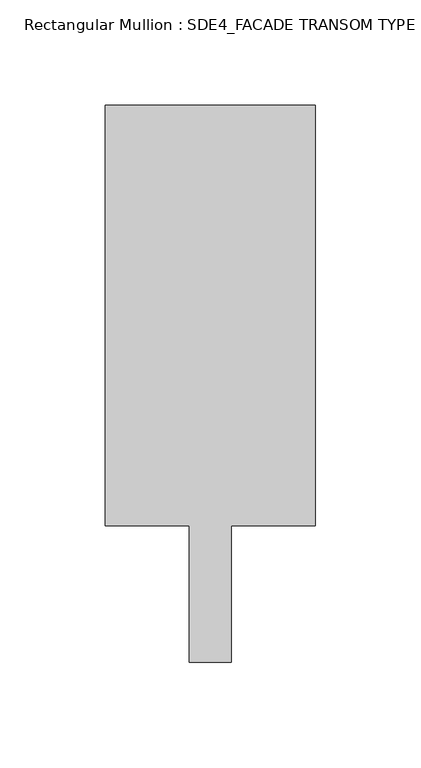
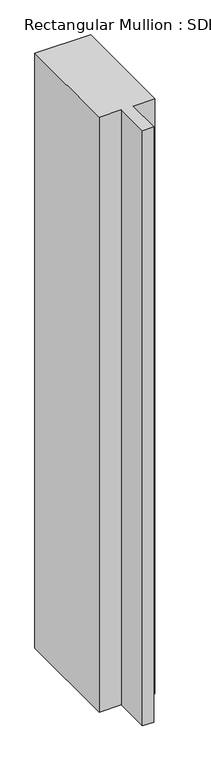
"""IFC4 building model written with IfcOpenShell, lengths in millimetres: member geometry, Rectangular Mullion : SDE4_FACADE TRANSOM TYPE 2."""

import ifcopenshell
import ifcopenshell.guid

model = None  # the IFC model being written
_history = None  # IfcOwnerHistory: only IFC2X3 demands one
_inside = {}  # id of a spatial element -> (the spatial element, [elements in it])
_under = {}  # id of a project, library or spatial element -> (it, [spatial elements below it])
_declared = {}  # id of a project -> (the project, [libraries it declares])
_typed = {}  # id of a type object -> (the type object, [elements of that type])
_made_of = {}  # id of a material, layer set ... -> (it, [elements and type objects made of it])


def new_model(schema):
    """Start an empty IFC model of exactly this schema.

    Asked for "IFC4X3", IfcOpenShell would pick the latest addendum, in which some entities
    have other attributes; the version numbers below select the first issue.
    IFC2X3 requires an IfcOwnerHistory on every rooted entity: one is made here for all.
    """
    global model, _history
    if schema == "IFC4X3":
        model = ifcopenshell.file(schema_version=(4, 3, 0, 0))
    else:
        model = ifcopenshell.file(schema=schema)
    _inside.clear()
    _under.clear()
    _declared.clear()
    _typed.clear()
    _made_of.clear()
    _history = None
    if model.schema == "IFC2X3":
        org = make("IfcOrganization", Name="unknown")
        user = make(
            "IfcPersonAndOrganization",
            ThePerson=make("IfcPerson", FamilyName="unknown"),
            TheOrganization=org,
        )
        app = make(
            "IfcApplication",
            ApplicationDeveloper=org,
            Version="unknown",
            ApplicationFullName="unknown",
            ApplicationIdentifier="unknown",
        )
        _history = make(
            "IfcOwnerHistory",
            OwningUser=user,
            OwningApplication=app,
            ChangeAction="ADDED",
            CreationDate=0,
        )
    return model


def make(cls, **values):
    """One entity of the class cls with the attributes given. An attribute that is None is left unset."""
    return model.create_entity(
        cls, **{name: value for name, value in values.items() if value is not None}
    )


def rooted(cls, **values):
    """An entity with a GlobalId (a new one), such as an element, a storey or a relation."""
    return make(cls, GlobalId=ifcopenshell.guid.new(), OwnerHistory=_history, **values)


def si_unit(unit_type, name, prefix=None):
    """IfcSIUnit, for example si_unit("LENGTHUNIT", "METRE", prefix="MILLI")."""
    return make("IfcSIUnit", UnitType=unit_type, Prefix=prefix, Name=name)


def assignment(units):
    """IfcUnitAssignment: the units of a project."""
    return None if units is None else make("IfcUnitAssignment", Units=units)


def point(xyz):
    """IfcCartesianPoint."""
    return None if xyz is None else make("IfcCartesianPoint", Coordinates=xyz)


def direction(xyz):
    """IfcDirection."""
    return None if xyz is None else make("IfcDirection", DirectionRatios=xyz)


def frame(location, z_axis=None, x_axis=None):
    """IfcAxis2Placement3D, a coordinate frame: its origin and axes. An axis left out is left unset."""
    return make(
        "IfcAxis2Placement3D",
        Location=point(location),
        Axis=direction(z_axis),
        RefDirection=direction(x_axis),
    )


def origin():
    """The frame at (0, 0, 0) with its axes left unset."""
    return frame((0.0, 0.0, 0.0))


def place(relative_to, where):
    """IfcLocalPlacement: puts the frame where relative to a parent placement (None: the world)."""
    return make(
        "IfcLocalPlacement", PlacementRelTo=relative_to, RelativePlacement=where
    )


def context(
    kind, dimensions, precision=None, world=None, true_north=None, identifier=None
):
    """IfcGeometricRepresentationContext, for example the 3D "Model" context."""
    return make(
        "IfcGeometricRepresentationContext",
        ContextIdentifier=identifier,
        ContextType=kind,
        CoordinateSpaceDimension=dimensions,
        Precision=precision,
        WorldCoordinateSystem=world,
        TrueNorth=true_north,
    )


def project(units=None, contexts=None):
    """IfcProject with its units and contexts."""
    return rooted(
        "IfcProject",
        Name="project",
        RepresentationContexts=contexts,
        UnitsInContext=assignment(units),
    )


def spatial(cls, under=None, at=None, **own):
    """A site, building, storey or space (cls), placed at a placement, below another one or the project."""
    s = rooted(cls, ObjectPlacement=at, **own)
    if under is not None:
        _under.setdefault(under.id(), (under, []))[1].append(s)
    return s


def polyline(points):
    """IfcPolyline through the points."""
    return make("IfcPolyline", Points=[point(p) for p in points])


def outline(outer, holes=None, kind="AREA"):
    """IfcArbitraryClosedProfileDef: a profile drawn as a closed curve; with holes, ...WithVoids."""
    if holes is None:
        return make("IfcArbitraryClosedProfileDef", ProfileType=kind, OuterCurve=outer)
    return make(
        "IfcArbitraryProfileDefWithVoids",
        ProfileType=kind,
        OuterCurve=outer,
        InnerCurves=holes,
    )


def extrude(swept, where, along, depth):
    """IfcExtrudedAreaSolid: the profile swept, set in the frame where, extruded along a direction by depth."""
    return make(
        "IfcExtrudedAreaSolid",
        SweptArea=swept,
        Position=where,
        ExtrudedDirection=direction(along),
        Depth=depth,
    )


def shape(context_of_items, identifier, shape_type, items):
    """IfcShapeRepresentation: the items that make up one representation, for example the "Body"."""
    return make(
        "IfcShapeRepresentation",
        ContextOfItems=context_of_items,
        RepresentationIdentifier=identifier,
        RepresentationType=shape_type,
        Items=items,
    )


def source(mapping_origin, context_of_items, identifier, shape_type, items):
    """IfcRepresentationMap: a shape defined once, which mapped items show again and again."""
    return make(
        "IfcRepresentationMap",
        MappingOrigin=mapping_origin,
        MappedRepresentation=shape(context_of_items, identifier, shape_type, items),
    )


def transform(
    local_origin,
    x_axis=None,
    y_axis=None,
    z_axis=None,
    scale=None,
    scale2=None,
    scale3=None,
    uniform=True,
):
    """IfcCartesianTransformationOperator3D, or its non-uniform kind. x_axis, y_axis, z_axis: its Axis1, 2, 3."""
    if uniform:
        return make(
            "IfcCartesianTransformationOperator3D",
            Axis1=direction(x_axis),
            Axis2=direction(y_axis),
            LocalOrigin=point(local_origin),
            Scale=scale,
            Axis3=direction(z_axis),
        )
    return make(
        "IfcCartesianTransformationOperator3DnonUniform",
        Axis1=direction(x_axis),
        Axis2=direction(y_axis),
        LocalOrigin=point(local_origin),
        Scale=scale,
        Axis3=direction(z_axis),
        Scale2=scale2,
        Scale3=scale3,
    )


def mapped(mapping_source, mapping_target):
    """IfcMappedItem: shows the shape of a source again, moved by a transform."""
    return make(
        "IfcMappedItem", MappingSource=mapping_source, MappingTarget=mapping_target
    )


def made_of(thing, what):
    """Note that an element or type object is made of a material, layer set ...; save() writes the relation."""
    if what is not None:
        _made_of.setdefault(what.id(), (what, []))[1].append(thing)
    return thing


def element(
    cls,
    number,
    at=None,
    inside=None,
    cuts=None,
    type_object=None,
    material=None,
    context=None,
    identifier="Body",
    shape_type=None,
    held_by="IfcProductDefinitionShape",
    body=None,
    shapes=None,
    **own,
):
    """One element of the class cls, such as IfcWall. Its Tag is "e" and its number.

    at: its placement. inside: the storey or other place that contains it. cuts: it is an
    opening in that element (IfcRelVoidsElement). A single representation is given by context,
    identifier, shape_type and body (its items); several are given by shapes. held_by: the class
    of the entity that holds the representations. save() writes the other relations.
    """
    e = rooted(cls, Tag="e%d" % number, ObjectPlacement=at, **own)
    if body is not None:
        shapes = [shape(context, identifier, shape_type, body)]
    if shapes is not None:
        e.Representation = make(held_by, Representations=shapes)
    if inside is not None:
        _inside.setdefault(inside.id(), (inside, []))[1].append(e)
    if cuts is not None:
        rooted(
            "IfcRelVoidsElement", RelatingBuildingElement=cuts, RelatedOpeningElement=e
        )
    if type_object is not None:
        _typed.setdefault(type_object.id(), (type_object, []))[1].append(e)
    return made_of(e, material)


def aggregate(whole, parts):
    """IfcRelAggregates: a whole, such as a stair, and the parts it consists of."""
    return rooted("IfcRelAggregates", RelatingObject=whole, RelatedObjects=parts)


def save(model, path):
    """Write the relations noted so far, then the file.

    IfcRelAggregates (storeys below a building ...), IfcRelContainedInSpatialStructure (elements
    in a storey), IfcRelDefinesByType, IfcRelAssociatesMaterial and IfcRelDeclares: one each for
    every whole, place, type object, material and project.
    """
    for whole, parts in _under.values():
        aggregate(whole, parts)
    for where, things in _inside.values():
        rooted(
            "IfcRelContainedInSpatialStructure",
            RelatedElements=things,
            RelatingStructure=where,
        )
    for kind, things in _typed.values():
        rooted("IfcRelDefinesByType", RelatedObjects=things, RelatingType=kind)
    for what, things in _made_of.values():
        rooted("IfcRelAssociatesMaterial", RelatedObjects=things, RelatingMaterial=what)
    for by, libraries in _declared.values():
        rooted("IfcRelDeclares", RelatingContext=by, RelatedDefinitions=libraries)
    model.write(path)


def rectangular_mullion_sde4_facade_transom_type_2_595efa1b(model_context):
    return source(origin(), model_context, "Body", "SweptSolid", [
        extrude(outline(polyline([(50.0, 132.5), (50.0, -67.5), (10.0, -67.5), (10.0, -132.5), (-10.0, -132.5), (-10.0, -67.5), (-50.0, -67.5), (-50.0, 132.5), (50.0, 132.5)])), frame((0.0, 0.0, -1129.8651301), z_axis=(0.0, 0.0, 1.0), x_axis=(1.0, 0.0, 0.0)), (0.0, 0.0, 1.0), 1129.8651301),
    ])


if __name__ == "__main__":
    model = new_model("IFC4")
    model_context = context("Model", 3, world=origin())
    ifc_project = project(units=[si_unit("LENGTHUNIT", "METRE", prefix="MILLI")], contexts=[model_context])
    site = spatial("IfcSite", under=ifc_project)
    building = spatial("IfcBuilding", under=site)
    placement = place(None, origin())
    rectangular_mullion_sde4_facade_transom_type_2_shape = rectangular_mullion_sde4_facade_transom_type_2_595efa1b(model_context)
    element("IfcMember", 1, ObjectType="Rectangular Mullion : SDE4_FACADE TRANSOM TYPE 2", at=placement, inside=building, context=model_context, shape_type="MappedRepresentation", body=[
        mapped(rectangular_mullion_sde4_facade_transom_type_2_shape, transform((0.0, 0.0, 0.0), x_axis=(1.0, 0.0, 0.0), y_axis=(0.0, 1.0, 0.0), z_axis=(0.0, 0.0, 1.0))),
    ])
    save(model, "model.ifc")

# Revit data of these elements
# Type "Rectangular Mullion : SDE4_FACADE TRANSOM TYPE 2"
#   built-in parameter 1007322 = 0.869423 (stored number, unit not read)
#   built-in parameter 1007321 = 0.164042 (stored number, unit not read)
#   built-in parameter 1007320 = 0.164042 (stored number, unit not read)
